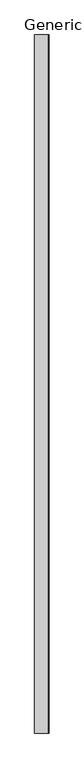
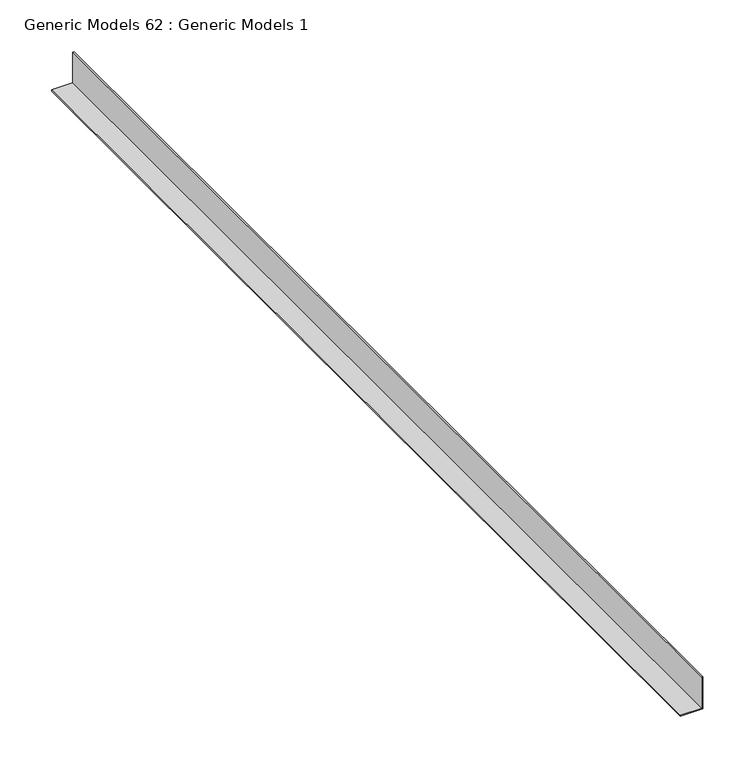
"""IFC4 building model written with IfcOpenShell, lengths in millimetres: proxy geometry, Generic Models 62 : Generic Models 1."""

from ifc_helpers import new_model, si_unit, frame, origin, place, context, project, spatial, polyline, outline, extrude, source, transform, mapped, element, save


def generic_models_62_generic_models_1_528f8659(model_context):
    return source(origin(), model_context, "Body", "SweptSolid", [
        extrude(outline(polyline([(2277.1204978, 51991.1377541), (2277.1204978, 51989.5502541), (2240.6079978, 51989.5502541), (2240.6079978, 51965.7377541), (2239.0204978, 51965.7377541), (2239.0204978, 51991.1377541), (2277.1204978, 51991.1377541)])), frame((0.0, 0.0, 0.0), z_axis=(0.0, 1.0, 0.0), x_axis=(0.0, 0.0, 1.0)), (0.0, 0.0, 1.0), 1219.2),
    ])


if __name__ == "__main__":
    model = new_model("IFC4")
    model_context = context("Model", 3, world=origin())
    ifc_project = project(units=[si_unit("LENGTHUNIT", "METRE", prefix="MILLI")], contexts=[model_context])
    site = spatial("IfcSite", under=ifc_project)
    building = spatial("IfcBuilding", under=site)
    placement = place(None, origin())
    generic_models_62_generic_models_1_shape = generic_models_62_generic_models_1_528f8659(model_context)
    element("IfcBuildingElementProxy", 1, Name="Generic Models 62 : Generic Models 1", ObjectType="Generic Models 62 : Generic Models 1", at=placement, inside=building, context=model_context, shape_type="MappedRepresentation", body=[
        mapped(generic_models_62_generic_models_1_shape, transform((0.0, 0.0, 0.0), x_axis=(1.0, 0.0, 0.0), y_axis=(0.0, 1.0, 0.0), z_axis=(0.0, 0.0, 1.0))),
    ])
    save(model, "model.ifc")

# Revit data of these elements
# Element 1 (IfcBuildingElementProxy, "Generic Models 62 : Generic Models 1")
#   Materials on its faces: "CEILING TRACK AS SCHEDULED"
# Materials
#   "CEILING TRACK AS SCHEDULED": class "Unassigned", colour RGB 210 209 208, transparency 0, Keynote = "M05121300.02", Cost = 0
